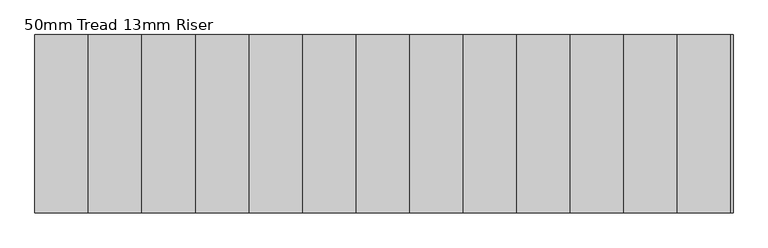
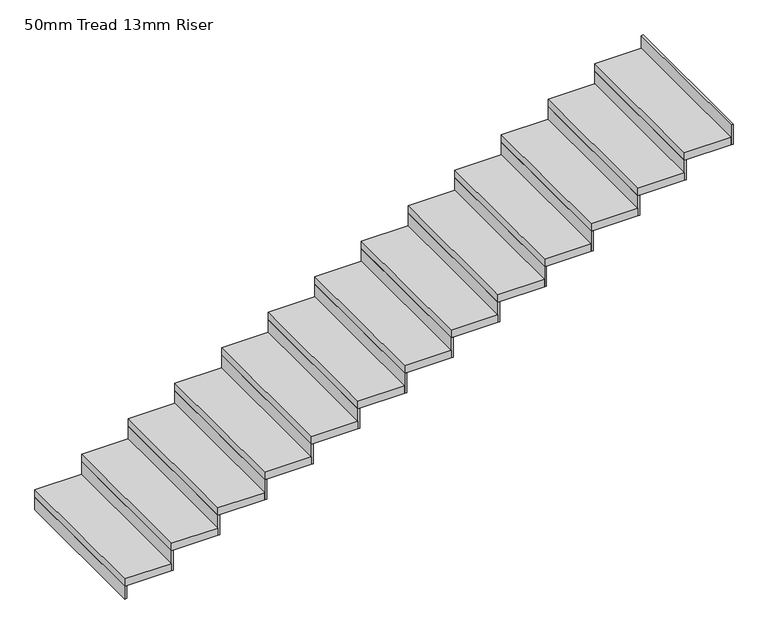
"""IFC4 building model written with IfcOpenShell, lengths in millimetres: stair flight geometry, 50mm Tread 13mm Riser."""

from ifc_helpers import new_model, si_unit, frame, origin, origin_with_axes, place, context, project, spatial, polyline, outline, extrude, source, transform, mapped, element, save


def stair_flight_50mm_tread_13mm_riser_3b11f18b(model_context):
    return source(origin(), model_context, "Body", "SweptSolid", [
        extrude(outline(polyline([(17642.336337, -4576.2808257), (17629.836337, -4576.2808257), (17629.836337, -3576.2808257), (17642.336337, -3576.2808257), (17642.336337, -4576.2808257)])), origin_with_axes(), (0.0, 0.0, 1.0), 86.3636364),
        extrude(outline(polyline([(17929.836337, -3576.2808257), (17929.836337, -4576.2808257), (17629.836337, -4576.2808257), (17629.836337, -3576.2808257), (17929.836337, -3576.2808257)])), frame((0.0, 0.0, 86.3636364), z_axis=(0.0, 0.0, 1.0), x_axis=(1.0, 0.0, 0.0)), (0.0, 0.0, 1.0), 50.0),
        extrude(outline(polyline([(17942.336337, -4576.2808257), (17929.836337, -4576.2808257), (17929.836337, -3576.2808257), (17942.336337, -3576.2808257), (17942.336337, -4576.2808257)])), frame((0.0, 0.0, 86.3636364), z_axis=(0.0, 0.0, 1.0), x_axis=(1.0, 0.0, 0.0)), (0.0, 0.0, 1.0), 136.3636364),
        extrude(outline(polyline([(18229.836337, -3576.2808257), (18229.836337, -4576.2808257), (17929.836337, -4576.2808257), (17929.836337, -3576.2808257), (18229.836337, -3576.2808257)])), frame((0.0, 0.0, 222.7272727), z_axis=(0.0, 0.0, 1.0), x_axis=(1.0, 0.0, 0.0)), (0.0, 0.0, 1.0), 50.0),
        extrude(outline(polyline([(18242.336337, -4576.2808257), (18229.836337, -4576.2808257), (18229.836337, -3576.2808257), (18242.336337, -3576.2808257), (18242.336337, -4576.2808257)])), frame((0.0, 0.0, 222.7272727), z_axis=(0.0, 0.0, 1.0), x_axis=(1.0, 0.0, 0.0)), (0.0, 0.0, 1.0), 136.3636364),
        extrude(outline(polyline([(18529.836337, -3576.2808257), (18529.836337, -4576.2808257), (18229.836337, -4576.2808257), (18229.836337, -3576.2808257), (18529.836337, -3576.2808257)])), frame((0.0, 0.0, 359.0909091), z_axis=(0.0, 0.0, 1.0), x_axis=(1.0, 0.0, 0.0)), (0.0, 0.0, 1.0), 50.0),
        extrude(outline(polyline([(18542.336337, -4576.2808257), (18529.836337, -4576.2808257), (18529.836337, -3576.2808257), (18542.336337, -3576.2808257), (18542.336337, -4576.2808257)])), frame((0.0, 0.0, 359.0909091), z_axis=(0.0, 0.0, 1.0), x_axis=(1.0, 0.0, 0.0)), (0.0, 0.0, 1.0), 136.3636364),
        extrude(outline(polyline([(18829.836337, -3576.2808257), (18829.836337, -4576.2808257), (18529.836337, -4576.2808257), (18529.836337, -3576.2808257), (18829.836337, -3576.2808257)])), frame((0.0, 0.0, 495.4545455), z_axis=(0.0, 0.0, 1.0), x_axis=(1.0, 0.0, 0.0)), (0.0, 0.0, 1.0), 50.0),
        extrude(outline(polyline([(18842.336337, -4576.2808257), (18829.836337, -4576.2808257), (18829.836337, -3576.2808257), (18842.336337, -3576.2808257), (18842.336337, -4576.2808257)])), frame((0.0, 0.0, 495.4545455), z_axis=(0.0, 0.0, 1.0), x_axis=(1.0, 0.0, 0.0)), (0.0, 0.0, 1.0), 136.3636364),
        extrude(outline(polyline([(19129.836337, -3576.2808257), (19129.836337, -4576.2808257), (18829.836337, -4576.2808257), (18829.836337, -3576.2808257), (19129.836337, -3576.2808257)])), frame((0.0, 0.0, 631.8181818), z_axis=(0.0, 0.0, 1.0), x_axis=(1.0, 0.0, 0.0)), (0.0, 0.0, 1.0), 50.0),
        extrude(outline(polyline([(19142.336337, -4576.2808257), (19129.836337, -4576.2808257), (19129.836337, -3576.2808257), (19142.336337, -3576.2808257), (19142.336337, -4576.2808257)])), frame((0.0, 0.0, 631.8181818), z_axis=(0.0, 0.0, 1.0), x_axis=(1.0, 0.0, 0.0)), (0.0, 0.0, 1.0), 136.3636364),
        extrude(outline(polyline([(19429.836337, -3576.2808257), (19429.836337, -4576.2808257), (19129.836337, -4576.2808257), (19129.836337, -3576.2808257), (19429.836337, -3576.2808257)])), frame((0.0, 0.0, 768.1818182), z_axis=(0.0, 0.0, 1.0), x_axis=(1.0, 0.0, 0.0)), (0.0, 0.0, 1.0), 50.0),
        extrude(outline(polyline([(19442.336337, -4576.2808257), (19429.836337, -4576.2808257), (19429.836337, -3576.2808257), (19442.336337, -3576.2808257), (19442.336337, -4576.2808257)])), frame((0.0, 0.0, 768.1818182), z_axis=(0.0, 0.0, 1.0), x_axis=(1.0, 0.0, 0.0)), (0.0, 0.0, 1.0), 136.3636364),
        extrude(outline(polyline([(19729.836337, -3576.2808257), (19729.836337, -4576.2808257), (19429.836337, -4576.2808257), (19429.836337, -3576.2808257), (19729.836337, -3576.2808257)])), frame((0.0, 0.0, 904.5454545), z_axis=(0.0, 0.0, 1.0), x_axis=(1.0, 0.0, 0.0)), (0.0, 0.0, 1.0), 50.0),
        extrude(outline(polyline([(19742.336337, -4576.2808257), (19729.836337, -4576.2808257), (19729.836337, -3576.2808257), (19742.336337, -3576.2808257), (19742.336337, -4576.2808257)])), frame((0.0, 0.0, 904.5454545), z_axis=(0.0, 0.0, 1.0), x_axis=(1.0, 0.0, 0.0)), (0.0, 0.0, 1.0), 136.3636364),
        extrude(outline(polyline([(20029.836337, -3576.2808257), (20029.836337, -4576.2808257), (19729.836337, -4576.2808257), (19729.836337, -3576.2808257), (20029.836337, -3576.2808257)])), frame((0.0, 0.0, 1040.9090909), z_axis=(0.0, 0.0, 1.0), x_axis=(1.0, 0.0, 0.0)), (0.0, 0.0, 1.0), 50.0),
        extrude(outline(polyline([(20042.336337, -4576.2808257), (20029.836337, -4576.2808257), (20029.836337, -3576.2808257), (20042.336337, -3576.2808257), (20042.336337, -4576.2808257)])), frame((0.0, 0.0, 1040.9090909), z_axis=(0.0, 0.0, 1.0), x_axis=(1.0, 0.0, 0.0)), (0.0, 0.0, 1.0), 136.3636364),
        extrude(outline(polyline([(20329.836337, -3576.2808257), (20329.836337, -4576.2808257), (20029.836337, -4576.2808257), (20029.836337, -3576.2808257), (20329.836337, -3576.2808257)])), frame((0.0, 0.0, 1177.2727273), z_axis=(0.0, 0.0, 1.0), x_axis=(1.0, 0.0, 0.0)), (0.0, 0.0, 1.0), 50.0),
        extrude(outline(polyline([(20342.336337, -4576.2808257), (20329.836337, -4576.2808257), (20329.836337, -3576.2808257), (20342.336337, -3576.2808257), (20342.336337, -4576.2808257)])), frame((0.0, 0.0, 1177.2727273), z_axis=(0.0, 0.0, 1.0), x_axis=(1.0, 0.0, 0.0)), (0.0, 0.0, 1.0), 136.3636364),
        extrude(outline(polyline([(20629.836337, -3576.2808257), (20629.836337, -4576.2808257), (20329.836337, -4576.2808257), (20329.836337, -3576.2808257), (20629.836337, -3576.2808257)])), frame((0.0, 0.0, 1313.6363636), z_axis=(0.0, 0.0, 1.0), x_axis=(1.0, 0.0, 0.0)), (0.0, 0.0, 1.0), 50.0),
        extrude(outline(polyline([(20642.336337, -4576.2808257), (20629.836337, -4576.2808257), (20629.836337, -3576.2808257), (20642.336337, -3576.2808257), (20642.336337, -4576.2808257)])), frame((0.0, 0.0, 1313.6363636), z_axis=(0.0, 0.0, 1.0), x_axis=(1.0, 0.0, 0.0)), (0.0, 0.0, 1.0), 136.3636364),
        extrude(outline(polyline([(20929.836337, -3576.2808257), (20929.836337, -4576.2808257), (20629.836337, -4576.2808257), (20629.836337, -3576.2808257), (20929.836337, -3576.2808257)])), frame((0.0, 0.0, 1450.0), z_axis=(0.0, 0.0, 1.0), x_axis=(1.0, 0.0, 0.0)), (0.0, 0.0, 1.0), 50.0),
        extrude(outline(polyline([(20942.336337, -4576.2808257), (20929.836337, -4576.2808257), (20929.836337, -3576.2808257), (20942.336337, -3576.2808257), (20942.336337, -4576.2808257)])), frame((0.0, 0.0, 1450.0), z_axis=(0.0, 0.0, 1.0), x_axis=(1.0, 0.0, 0.0)), (0.0, 0.0, 1.0), 136.3636364),
        extrude(outline(polyline([(21229.836337, -3576.2808257), (21229.836337, -4576.2808257), (20929.836337, -4576.2808257), (20929.836337, -3576.2808257), (21229.836337, -3576.2808257)])), frame((0.0, 0.0, 1586.3636364), z_axis=(0.0, 0.0, 1.0), x_axis=(1.0, 0.0, 0.0)), (0.0, 0.0, 1.0), 50.0),
        extrude(outline(polyline([(21242.336337, -4576.2808257), (21229.836337, -4576.2808257), (21229.836337, -3576.2808257), (21242.336337, -3576.2808257), (21242.336337, -4576.2808257)])), frame((0.0, 0.0, 1586.3636364), z_axis=(0.0, 0.0, 1.0), x_axis=(1.0, 0.0, 0.0)), (0.0, 0.0, 1.0), 136.3636364),
        extrude(outline(polyline([(21542.336337, -4576.2808257), (21529.836337, -4576.2808257), (21529.836337, -3576.2808257), (21542.336337, -3576.2808257), (21542.336337, -4576.2808257)])), frame((0.0, 0.0, 1722.7272727), z_axis=(0.0, 0.0, 1.0), x_axis=(1.0, 0.0, 0.0)), (0.0, 0.0, 1.0), 136.3636364),
        extrude(outline(polyline([(21529.836337, -3576.2808257), (21529.836337, -4576.2808257), (21229.836337, -4576.2808257), (21229.836337, -3576.2808257), (21529.836337, -3576.2808257)])), frame((0.0, 0.0, 1722.7272727), z_axis=(0.0, 0.0, 1.0), x_axis=(1.0, 0.0, 0.0)), (0.0, 0.0, 1.0), 50.0),
    ])


if __name__ == "__main__":
    model = new_model("IFC4")
    model_context = context("Model", 3, world=origin())
    ifc_project = project(units=[si_unit("LENGTHUNIT", "METRE", prefix="MILLI")], contexts=[model_context])
    site = spatial("IfcSite", under=ifc_project)
    building = spatial("IfcBuilding", under=site)
    placement = place(None, origin())
    stair_flight_50mm_tread_13mm_riser_shape = stair_flight_50mm_tread_13mm_riser_3b11f18b(model_context)
    element("IfcStairFlight", 1, ObjectType="50mm Tread 13mm Riser", at=placement, inside=building, context=model_context, shape_type="MappedRepresentation", body=[
        mapped(stair_flight_50mm_tread_13mm_riser_shape, transform((0.0, 0.0, 0.0), x_axis=(1.0, 0.0, 0.0), y_axis=(0.0, 1.0, 0.0), z_axis=(0.0, 0.0, 1.0))),
    ])
    save(model, "model.ifc")
